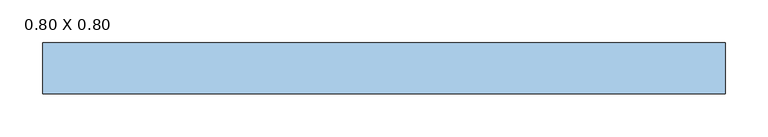
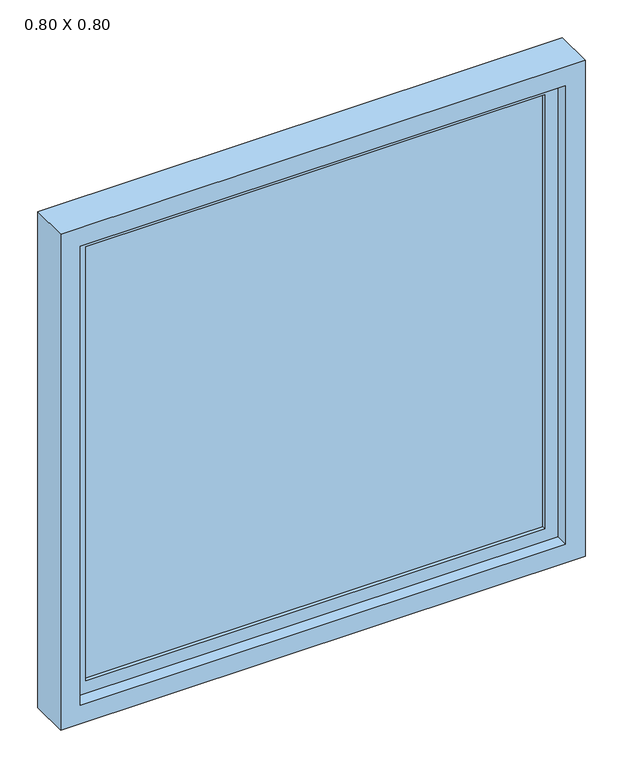
"""IFC4 building model written with IfcOpenShell, lengths in millimetres: window geometry, JANELA_MAXIM-AR_VIDRO : 0.80 X 0.80."""

from ifc_helpers import new_model, si_unit, frame, origin, place, context, project, spatial, polyline, outline, extrude, source, transform, mapped, element, save


def window_0_80_x_0_80_29a19849(model_context):
    return source(origin(), model_context, "Body", "SweptSolid", [
        extrude(outline(polyline([(-350.0, 4.0), (350.0, 4.0), (350.0, -4.0), (-350.0, -4.0), (-350.0, 4.0)])), frame((0.0, 0.0, 1550.0), z_axis=(0.0, 0.0, 1.0), x_axis=(1.0, 0.0, 0.0)), (0.0, 0.0, 1.0), 700.0),
        extrude(outline(polyline([(1530.0, 370.0), (2270.0, 370.0), (2270.0, -370.0), (1530.0, -370.0), (1530.0, 370.0)]), holes=[polyline([(2250.0, 350.0), (1550.0, 350.0), (1550.0, -350.0), (2250.0, -350.0), (2250.0, 350.0)])]), frame((0.0, -10.0, 0.0), z_axis=(0.0, 1.0, 0.0), x_axis=(0.0, 0.0, 1.0)), (0.0, 0.0, 1.0), 20.0),
        extrude(outline(polyline([(2300.0, 400.0), (2300.0, -400.0), (1500.0, -400.0), (1500.0, 400.0), (2300.0, 400.0)]), holes=[polyline([(1530.0, 370.0), (1530.0, -370.0), (2270.0, -370.0), (2270.0, 370.0), (1530.0, 370.0)])]), frame((0.0, -30.0, 0.0), z_axis=(0.0, 1.0, 0.0), x_axis=(0.0, 0.0, 1.0)), (0.0, 0.0, 1.0), 60.0),
    ])


if __name__ == "__main__":
    model = new_model("IFC4")
    model_context = context("Model", 3, world=origin())
    ifc_project = project(units=[si_unit("LENGTHUNIT", "METRE", prefix="MILLI")], contexts=[model_context])
    site = spatial("IfcSite", under=ifc_project)
    building = spatial("IfcBuilding", under=site)
    placement = place(None, origin())
    window_0_80_x_0_80_shape = window_0_80_x_0_80_29a19849(model_context)
    element("IfcWindow", 1, ObjectType="JANELA_MAXIM-AR_VIDRO : 0.80 X 0.80", at=placement, inside=building, context=model_context, shape_type="MappedRepresentation", body=[
        mapped(window_0_80_x_0_80_shape, transform((0.0, 0.0, 0.0), x_axis=(1.0, 0.0, 0.0), y_axis=(0.0, 1.0, 0.0), z_axis=(0.0, 0.0, 1.0))),
    ])
    save(model, "model.ifc")

# Revit data of these elements
# Type "JANELA_MAXIM-AR_VIDRO : 0.80 X 0.80"
#   Type Mark = "J5"
#   Largura Painel [instance default] = 0.02 m
#   Largura Esquadria [instance default] = 0.06 m
#   Espessura Vidro [instance default] = 0.008 m
#   Espessura Painel [instance default] = 0.02 m
#   Espessura Esquadria [instance default] = 0.03 m
#   Height = 0.80 m
#   Altura-padrão do peitoril = 1.50 m
#   Width = 0.80 m
#   Vidro = .VIDRO
#   Esquadria = .ALUMÍNIO COM PINTURA ELETROSTÁTICA BRANCA
#   Wall Closure = (empty or 0)
# Element 1 (IfcWindow, "JANELA_MAXIM-AR_VIDRO : 0.80 X 0.80")
#   Materials on its faces: ".ALUMÍNIO COM PINTURA ELETROSTÁTICA BRANCA", ".VIDRO"
# Materials
#   ".VIDRO": class "Genérico", colour RGB 198 236 255, transparency 0.95, Cost = 0
#   ".ALUMÍNIO COM PINTURA ELETROSTÁTICA BRANCA": class "CC_METAIS", colour RGB 241 241 241, transparency 0, Cost = 0
